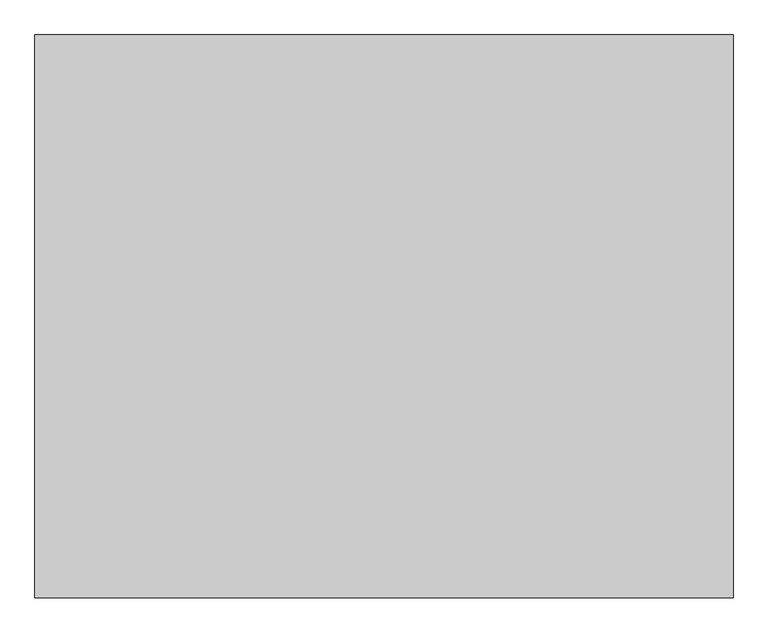
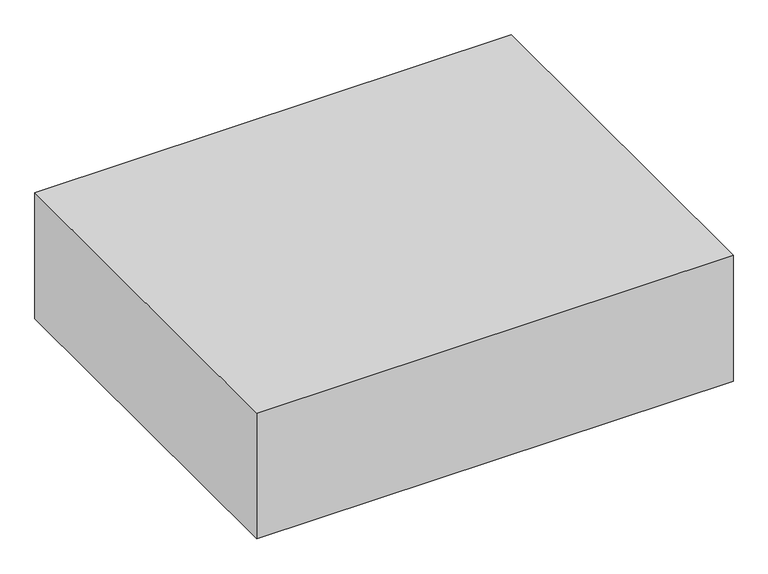
"""IFC4 building model written with IfcOpenShell, lengths in millimetres: proxy geometry, Space Planning Box_hec : Space Planning Box_hec."""

import ifcopenshell
import ifcopenshell.guid

model = None  # the IFC model being written
_history = None  # IfcOwnerHistory: only IFC2X3 demands one
_inside = {}  # id of a spatial element -> (the spatial element, [elements in it])
_under = {}  # id of a project, library or spatial element -> (it, [spatial elements below it])
_declared = {}  # id of a project -> (the project, [libraries it declares])
_typed = {}  # id of a type object -> (the type object, [elements of that type])
_made_of = {}  # id of a material, layer set ... -> (it, [elements and type objects made of it])


def new_model(schema):
    """Start an empty IFC model of exactly this schema.

    Asked for "IFC4X3", IfcOpenShell would pick the latest addendum, in which some entities
    have other attributes; the version numbers below select the first issue.
    IFC2X3 requires an IfcOwnerHistory on every rooted entity: one is made here for all.
    """
    global model, _history
    if schema == "IFC4X3":
        model = ifcopenshell.file(schema_version=(4, 3, 0, 0))
    else:
        model = ifcopenshell.file(schema=schema)
    _inside.clear()
    _under.clear()
    _declared.clear()
    _typed.clear()
    _made_of.clear()
    _history = None
    if model.schema == "IFC2X3":
        org = make("IfcOrganization", Name="unknown")
        user = make(
            "IfcPersonAndOrganization",
            ThePerson=make("IfcPerson", FamilyName="unknown"),
            TheOrganization=org,
        )
        app = make(
            "IfcApplication",
            ApplicationDeveloper=org,
            Version="unknown",
            ApplicationFullName="unknown",
            ApplicationIdentifier="unknown",
        )
        _history = make(
            "IfcOwnerHistory",
            OwningUser=user,
            OwningApplication=app,
            ChangeAction="ADDED",
            CreationDate=0,
        )
    return model


def make(cls, **values):
    """One entity of the class cls with the attributes given. An attribute that is None is left unset."""
    return model.create_entity(
        cls, **{name: value for name, value in values.items() if value is not None}
    )


def rooted(cls, **values):
    """An entity with a GlobalId (a new one), such as an element, a storey or a relation."""
    return make(cls, GlobalId=ifcopenshell.guid.new(), OwnerHistory=_history, **values)


def si_unit(unit_type, name, prefix=None):
    """IfcSIUnit, for example si_unit("LENGTHUNIT", "METRE", prefix="MILLI")."""
    return make("IfcSIUnit", UnitType=unit_type, Prefix=prefix, Name=name)


def assignment(units):
    """IfcUnitAssignment: the units of a project."""
    return None if units is None else make("IfcUnitAssignment", Units=units)


def point(xyz):
    """IfcCartesianPoint."""
    return None if xyz is None else make("IfcCartesianPoint", Coordinates=xyz)


def direction(xyz):
    """IfcDirection."""
    return None if xyz is None else make("IfcDirection", DirectionRatios=xyz)


def frame(location, z_axis=None, x_axis=None):
    """IfcAxis2Placement3D, a coordinate frame: its origin and axes. An axis left out is left unset."""
    return make(
        "IfcAxis2Placement3D",
        Location=point(location),
        Axis=direction(z_axis),
        RefDirection=direction(x_axis),
    )


def origin():
    """The frame at (0, 0, 0) with its axes left unset."""
    return frame((0.0, 0.0, 0.0))


def origin_with_axes():
    """The frame at (0, 0, 0) with the z axis (0, 0, 1) and the x axis (1, 0, 0) written out."""
    return frame((0.0, 0.0, 0.0), z_axis=(0.0, 0.0, 1.0), x_axis=(1.0, 0.0, 0.0))


def place(relative_to, where):
    """IfcLocalPlacement: puts the frame where relative to a parent placement (None: the world)."""
    return make(
        "IfcLocalPlacement", PlacementRelTo=relative_to, RelativePlacement=where
    )


def context(
    kind, dimensions, precision=None, world=None, true_north=None, identifier=None
):
    """IfcGeometricRepresentationContext, for example the 3D "Model" context."""
    return make(
        "IfcGeometricRepresentationContext",
        ContextIdentifier=identifier,
        ContextType=kind,
        CoordinateSpaceDimension=dimensions,
        Precision=precision,
        WorldCoordinateSystem=world,
        TrueNorth=true_north,
    )


def project(units=None, contexts=None):
    """IfcProject with its units and contexts."""
    return rooted(
        "IfcProject",
        Name="project",
        RepresentationContexts=contexts,
        UnitsInContext=assignment(units),
    )


def spatial(cls, under=None, at=None, **own):
    """A site, building, storey or space (cls), placed at a placement, below another one or the project."""
    s = rooted(cls, ObjectPlacement=at, **own)
    if under is not None:
        _under.setdefault(under.id(), (under, []))[1].append(s)
    return s


def polyline(points):
    """IfcPolyline through the points."""
    return make("IfcPolyline", Points=[point(p) for p in points])


def outline(outer, holes=None, kind="AREA"):
    """IfcArbitraryClosedProfileDef: a profile drawn as a closed curve; with holes, ...WithVoids."""
    if holes is None:
        return make("IfcArbitraryClosedProfileDef", ProfileType=kind, OuterCurve=outer)
    return make(
        "IfcArbitraryProfileDefWithVoids",
        ProfileType=kind,
        OuterCurve=outer,
        InnerCurves=holes,
    )


def extrude(swept, where, along, depth):
    """IfcExtrudedAreaSolid: the profile swept, set in the frame where, extruded along a direction by depth."""
    return make(
        "IfcExtrudedAreaSolid",
        SweptArea=swept,
        Position=where,
        ExtrudedDirection=direction(along),
        Depth=depth,
    )


def shape(context_of_items, identifier, shape_type, items):
    """IfcShapeRepresentation: the items that make up one representation, for example the "Body"."""
    return make(
        "IfcShapeRepresentation",
        ContextOfItems=context_of_items,
        RepresentationIdentifier=identifier,
        RepresentationType=shape_type,
        Items=items,
    )


def source(mapping_origin, context_of_items, identifier, shape_type, items):
    """IfcRepresentationMap: a shape defined once, which mapped items show again and again."""
    return make(
        "IfcRepresentationMap",
        MappingOrigin=mapping_origin,
        MappedRepresentation=shape(context_of_items, identifier, shape_type, items),
    )


def transform(
    local_origin,
    x_axis=None,
    y_axis=None,
    z_axis=None,
    scale=None,
    scale2=None,
    scale3=None,
    uniform=True,
):
    """IfcCartesianTransformationOperator3D, or its non-uniform kind. x_axis, y_axis, z_axis: its Axis1, 2, 3."""
    if uniform:
        return make(
            "IfcCartesianTransformationOperator3D",
            Axis1=direction(x_axis),
            Axis2=direction(y_axis),
            LocalOrigin=point(local_origin),
            Scale=scale,
            Axis3=direction(z_axis),
        )
    return make(
        "IfcCartesianTransformationOperator3DnonUniform",
        Axis1=direction(x_axis),
        Axis2=direction(y_axis),
        LocalOrigin=point(local_origin),
        Scale=scale,
        Axis3=direction(z_axis),
        Scale2=scale2,
        Scale3=scale3,
    )


def mapped(mapping_source, mapping_target):
    """IfcMappedItem: shows the shape of a source again, moved by a transform."""
    return make(
        "IfcMappedItem", MappingSource=mapping_source, MappingTarget=mapping_target
    )


def made_of(thing, what):
    """Note that an element or type object is made of a material, layer set ...; save() writes the relation."""
    if what is not None:
        _made_of.setdefault(what.id(), (what, []))[1].append(thing)
    return thing


def element(
    cls,
    number,
    at=None,
    inside=None,
    cuts=None,
    type_object=None,
    material=None,
    context=None,
    identifier="Body",
    shape_type=None,
    held_by="IfcProductDefinitionShape",
    body=None,
    shapes=None,
    **own,
):
    """One element of the class cls, such as IfcWall. Its Tag is "e" and its number.

    at: its placement. inside: the storey or other place that contains it. cuts: it is an
    opening in that element (IfcRelVoidsElement). A single representation is given by context,
    identifier, shape_type and body (its items); several are given by shapes. held_by: the class
    of the entity that holds the representations. save() writes the other relations.
    """
    e = rooted(cls, Tag="e%d" % number, ObjectPlacement=at, **own)
    if body is not None:
        shapes = [shape(context, identifier, shape_type, body)]
    if shapes is not None:
        e.Representation = make(held_by, Representations=shapes)
    if inside is not None:
        _inside.setdefault(inside.id(), (inside, []))[1].append(e)
    if cuts is not None:
        rooted(
            "IfcRelVoidsElement", RelatingBuildingElement=cuts, RelatedOpeningElement=e
        )
    if type_object is not None:
        _typed.setdefault(type_object.id(), (type_object, []))[1].append(e)
    return made_of(e, material)


def aggregate(whole, parts):
    """IfcRelAggregates: a whole, such as a stair, and the parts it consists of."""
    return rooted("IfcRelAggregates", RelatingObject=whole, RelatedObjects=parts)


def save(model, path):
    """Write the relations noted so far, then the file.

    IfcRelAggregates (storeys below a building ...), IfcRelContainedInSpatialStructure (elements
    in a storey), IfcRelDefinesByType, IfcRelAssociatesMaterial and IfcRelDeclares: one each for
    every whole, place, type object, material and project.
    """
    for whole, parts in _under.values():
        aggregate(whole, parts)
    for where, things in _inside.values():
        rooted(
            "IfcRelContainedInSpatialStructure",
            RelatedElements=things,
            RelatingStructure=where,
        )
    for kind, things in _typed.values():
        rooted("IfcRelDefinesByType", RelatedObjects=things, RelatingType=kind)
    for what, things in _made_of.values():
        rooted("IfcRelAssociatesMaterial", RelatedObjects=things, RelatingMaterial=what)
    for by, libraries in _declared.values():
        rooted("IfcRelDeclares", RelatingContext=by, RelatedDefinitions=libraries)
    model.write(path)


def generic_models_5fb19e15(model_context):
    return source(origin(), model_context, "Body", "SweptSolid", [
        extrude(outline(polyline([(9300.0, 7500.0), (9300.0, -7500.0), (-9300.0, -7500.0), (-9300.0, 7500.0), (9300.0, 7500.0)])), origin_with_axes(), (0.0, 0.0, 1.0), 5200.0),
    ])


if __name__ == "__main__":
    model = new_model("IFC4")
    model_context = context("Model", 3, world=origin())
    ifc_project = project(units=[si_unit("LENGTHUNIT", "METRE", prefix="MILLI")], contexts=[model_context])
    site = spatial("IfcSite", under=ifc_project)
    building = spatial("IfcBuilding", under=site)
    placement = place(None, origin())
    generic_models_shape = generic_models_5fb19e15(model_context)
    element("IfcBuildingElementProxy", 1, Name="Space Planning Box_hec : Space Planning Box_hec", ObjectType="Space Planning Box_hec : Space Planning Box_hec", at=placement, inside=building, context=model_context, shape_type="MappedRepresentation", body=[
        mapped(generic_models_shape, transform((0.0, 0.0, 0.0), x_axis=(1.0, 0.0, 0.0), y_axis=(0.0, 1.0, 0.0), z_axis=(0.0, 0.0, 1.0))),
    ])
    save(model, "model.ifc")

# Revit data of these elements
# Type "Space Planning Box_hec : Space Planning Box_hec"
#   Type Comments = "..."
#   Room Name [instance default] = "?"
#   Interior Finish [instance default] = ""
#   Exterior Finish [instance default] = ""
#   Department [instance default] = ""
#   Assembly Code = "..."
#   ceiling height [instance default] = 0
#   Width [instance default] = 1524 mm
#   Program Area [instance default] = 0.00 m²
#   Length [instance default] = 1524 mm
#   Height [instance default] = 1524 mm
#   Area [instance default] = 2.32258 m²
#   Fill Color [instance default] = Cyan
#   Default Elevation = 0
# Element 1 (IfcBuildingElementProxy, "Space Planning Box_hec : Space Planning Box_hec")
#   Room Name = "Electronic Room"
#   Interior Finish = "IW1..N/A,,WB2..N/A,,FL7..N/A,,CL4..N/A"
#   Exterior Finish = "N/A..N/A,,EW1..N/A"
#   Department = "CI"
#   ceiling height = 3000
#   Width = 18600 mm
#   Program Area = 279.00 m²
#   Length = 15000 mm
#   Height = 5200 mm
#   Area = 279.00 m²
#   Fill Color = Yellow
#   Materials on its faces: "Yellow"
# Materials
#   "Cyan": class "Generic", colour RGB 0 255 255, transparency 0.2, Cost = 0
#   "Yellow": class "Generic", colour RGB 255 255 0, transparency 0.2, Cost = 0
